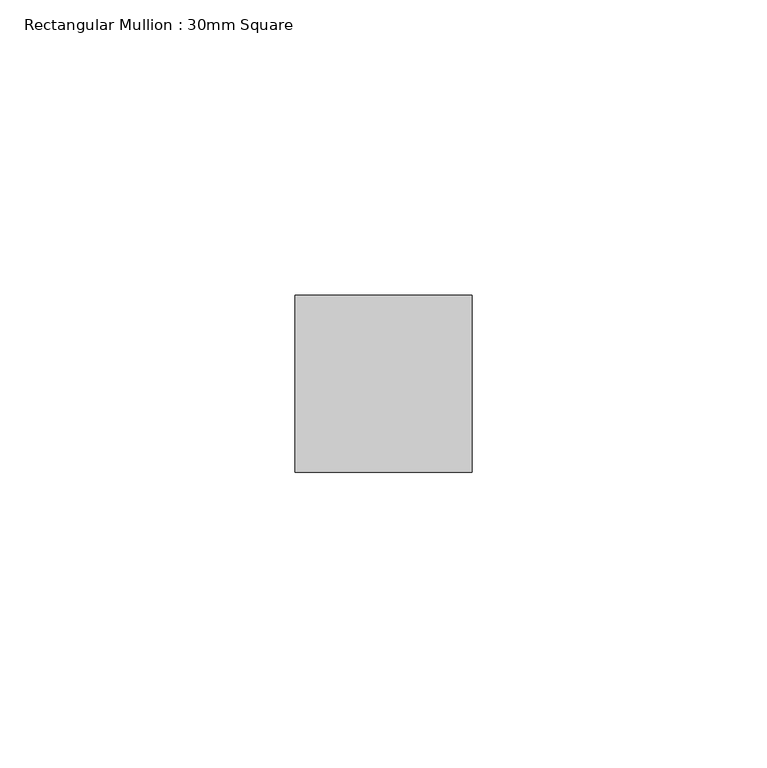
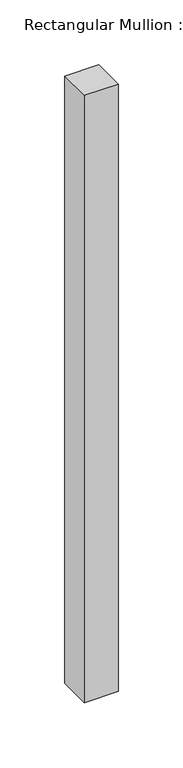
"""IFC4 building model written with IfcOpenShell, lengths in millimetres: member geometry, Rectangular Mullion : 30mm Square."""

from ifc_helpers import new_model, si_unit, frame, origin, place, context, project, spatial, polyline, outline, extrude, source, transform, mapped, element, save


def rectangular_mullion_30mm_square_a2b02fc3(model_context):
    return source(origin(), model_context, "Body", "SweptSolid", [
        extrude(outline(polyline([(15.0, 15.0), (15.0, -15.0), (-15.0, -15.0), (-15.0, 15.0), (15.0, 15.0)])), frame((0.0, 0.0, -571.5319572), z_axis=(0.0, 0.0, 1.0), x_axis=(1.0, 0.0, 0.0)), (0.0, 0.0, 1.0), 571.5319572),
    ])


if __name__ == "__main__":
    model = new_model("IFC4")
    model_context = context("Model", 3, world=origin())
    ifc_project = project(units=[si_unit("LENGTHUNIT", "METRE", prefix="MILLI")], contexts=[model_context])
    site = spatial("IfcSite", under=ifc_project)
    building = spatial("IfcBuilding", under=site)
    placement = place(None, origin())
    rectangular_mullion_30mm_square_shape = rectangular_mullion_30mm_square_a2b02fc3(model_context)
    element("IfcMember", 1, ObjectType="Rectangular Mullion : 30mm Square", at=placement, inside=building, context=model_context, shape_type="MappedRepresentation", body=[
        mapped(rectangular_mullion_30mm_square_shape, transform((0.0, 0.0, 0.0), x_axis=(1.0, 0.0, 0.0), y_axis=(0.0, 1.0, 0.0), z_axis=(0.0, 0.0, 1.0))),
    ])
    save(model, "model.ifc")

# Revit data of these elements
# Type "Rectangular Mullion : 30mm Square"
#   built-in parameter 1007304 = 0.0984252 (stored number, unit not read)
#   built-in parameter 1007301 = 0.0492126 (stored number, unit not read)
#   built-in parameter 1007300 = 0.0492126 (stored number, unit not read)
# Element 1 (IfcMember, "Rectangular Mullion : 30mm Square")
#   Materials on its faces: "Aluminum"
# Materials
#   "Aluminum": class "Metal", colour RGB 244 244 244, transparency 0, Description = "Aluminum 6061", Cost = 0
